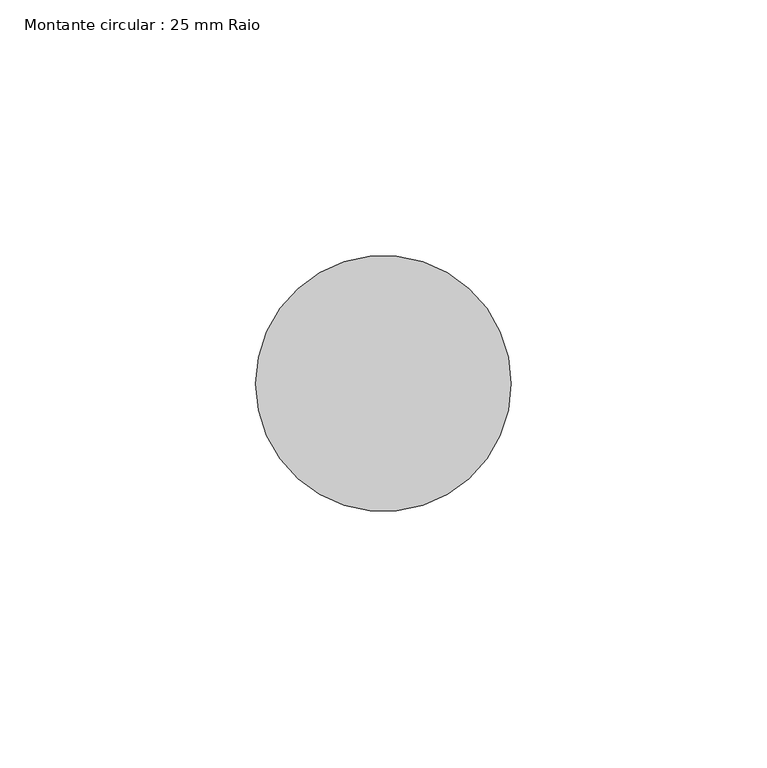
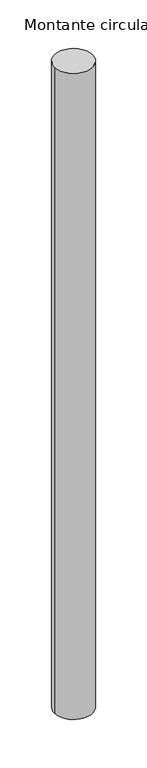
"""IFC4 building model written with IfcOpenShell, lengths in millimetres: member geometry, Montante circular : 25 mm Raio."""

from ifc_helpers import new_model, si_unit, point, frame, origin, origin_2d, place, context, project, spatial, circle_curve, trimmed, segment, composite_curve, outline, extrude, source, transform, mapped, element, save


def montante_circular_25_mm_raio_8ba79aec(model_context):
    return source(origin(), model_context, "Body", "SweptSolid", [
        extrude(outline(composite_curve([segment(trimmed(circle_curve(origin_2d(), 25.0), [point((25.0, 0.0))], [point((-25.0, 0.0))], False, "CARTESIAN"), True, "CONTINUOUS"), segment(trimmed(circle_curve(origin_2d(), 25.0), [point((-25.0, 0.0))], [point((25.0, 0.0))], False, "CARTESIAN"), True, "CONTINUOUS")], self_intersect=False)), frame((0.0, 0.0, -900.0), z_axis=(0.0, 0.0, 1.0), x_axis=(1.0, 0.0, 0.0)), (0.0, 0.0, 1.0), 900.0),
    ])


if __name__ == "__main__":
    model = new_model("IFC4")
    model_context = context("Model", 3, world=origin())
    ifc_project = project(units=[si_unit("LENGTHUNIT", "METRE", prefix="MILLI")], contexts=[model_context])
    site = spatial("IfcSite", under=ifc_project)
    building = spatial("IfcBuilding", under=site)
    placement = place(None, origin())
    montante_circular_25_mm_raio_shape = montante_circular_25_mm_raio_8ba79aec(model_context)
    element("IfcMember", 1, ObjectType="Montante circular : 25 mm Raio", at=placement, inside=building, context=model_context, shape_type="MappedRepresentation", body=[
        mapped(montante_circular_25_mm_raio_shape, transform((0.0, 0.0, 0.0), x_axis=(1.0, 0.0, 0.0), y_axis=(0.0, 1.0, 0.0), z_axis=(0.0, 0.0, 1.0))),
    ])
    save(model, "model.ifc")

# Revit data of these elements
# Type "Montante circular : 25 mm Raio"
#   built-in parameter 1007350 = 0.082021 (stored number, unit not read)
# Element 1 (IfcMember, "Montante circular : 25 mm Raio")
#   Materials on its faces: "Alumín."
# Materials
#   "Alumín.": class "Metal", colour RGB 247 247 247, transparency 0, Description = "Alumín. 6061", Cost = 0
